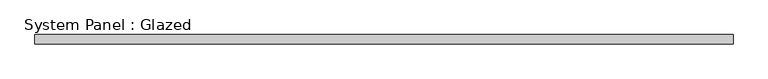
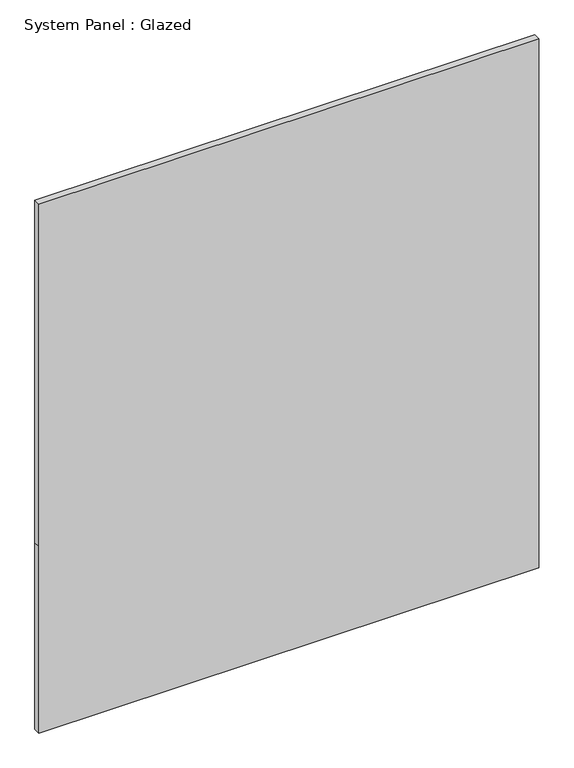
"""IFC4 building model written with IfcOpenShell, lengths in millimetres: plate geometry, System Panel : Glazed."""

import ifcopenshell
import ifcopenshell.guid

model = None  # the IFC model being written
_history = None  # IfcOwnerHistory: only IFC2X3 demands one
_inside = {}  # id of a spatial element -> (the spatial element, [elements in it])
_under = {}  # id of a project, library or spatial element -> (it, [spatial elements below it])
_declared = {}  # id of a project -> (the project, [libraries it declares])
_typed = {}  # id of a type object -> (the type object, [elements of that type])
_made_of = {}  # id of a material, layer set ... -> (it, [elements and type objects made of it])


def new_model(schema):
    """Start an empty IFC model of exactly this schema.

    Asked for "IFC4X3", IfcOpenShell would pick the latest addendum, in which some entities
    have other attributes; the version numbers below select the first issue.
    IFC2X3 requires an IfcOwnerHistory on every rooted entity: one is made here for all.
    """
    global model, _history
    if schema == "IFC4X3":
        model = ifcopenshell.file(schema_version=(4, 3, 0, 0))
    else:
        model = ifcopenshell.file(schema=schema)
    _inside.clear()
    _under.clear()
    _declared.clear()
    _typed.clear()
    _made_of.clear()
    _history = None
    if model.schema == "IFC2X3":
        org = make("IfcOrganization", Name="unknown")
        user = make(
            "IfcPersonAndOrganization",
            ThePerson=make("IfcPerson", FamilyName="unknown"),
            TheOrganization=org,
        )
        app = make(
            "IfcApplication",
            ApplicationDeveloper=org,
            Version="unknown",
            ApplicationFullName="unknown",
            ApplicationIdentifier="unknown",
        )
        _history = make(
            "IfcOwnerHistory",
            OwningUser=user,
            OwningApplication=app,
            ChangeAction="ADDED",
            CreationDate=0,
        )
    return model


def make(cls, **values):
    """One entity of the class cls with the attributes given. An attribute that is None is left unset."""
    return model.create_entity(
        cls, **{name: value for name, value in values.items() if value is not None}
    )


def rooted(cls, **values):
    """An entity with a GlobalId (a new one), such as an element, a storey or a relation."""
    return make(cls, GlobalId=ifcopenshell.guid.new(), OwnerHistory=_history, **values)


def si_unit(unit_type, name, prefix=None):
    """IfcSIUnit, for example si_unit("LENGTHUNIT", "METRE", prefix="MILLI")."""
    return make("IfcSIUnit", UnitType=unit_type, Prefix=prefix, Name=name)


def assignment(units):
    """IfcUnitAssignment: the units of a project."""
    return None if units is None else make("IfcUnitAssignment", Units=units)


def point(xyz):
    """IfcCartesianPoint."""
    return None if xyz is None else make("IfcCartesianPoint", Coordinates=xyz)


def direction(xyz):
    """IfcDirection."""
    return None if xyz is None else make("IfcDirection", DirectionRatios=xyz)


def frame(location, z_axis=None, x_axis=None):
    """IfcAxis2Placement3D, a coordinate frame: its origin and axes. An axis left out is left unset."""
    return make(
        "IfcAxis2Placement3D",
        Location=point(location),
        Axis=direction(z_axis),
        RefDirection=direction(x_axis),
    )


def origin():
    """The frame at (0, 0, 0) with its axes left unset."""
    return frame((0.0, 0.0, 0.0))


def place(relative_to, where):
    """IfcLocalPlacement: puts the frame where relative to a parent placement (None: the world)."""
    return make(
        "IfcLocalPlacement", PlacementRelTo=relative_to, RelativePlacement=where
    )


def context(
    kind, dimensions, precision=None, world=None, true_north=None, identifier=None
):
    """IfcGeometricRepresentationContext, for example the 3D "Model" context."""
    return make(
        "IfcGeometricRepresentationContext",
        ContextIdentifier=identifier,
        ContextType=kind,
        CoordinateSpaceDimension=dimensions,
        Precision=precision,
        WorldCoordinateSystem=world,
        TrueNorth=true_north,
    )


def project(units=None, contexts=None):
    """IfcProject with its units and contexts."""
    return rooted(
        "IfcProject",
        Name="project",
        RepresentationContexts=contexts,
        UnitsInContext=assignment(units),
    )


def spatial(cls, under=None, at=None, **own):
    """A site, building, storey or space (cls), placed at a placement, below another one or the project."""
    s = rooted(cls, ObjectPlacement=at, **own)
    if under is not None:
        _under.setdefault(under.id(), (under, []))[1].append(s)
    return s


def polyline(points):
    """IfcPolyline through the points."""
    return make("IfcPolyline", Points=[point(p) for p in points])


def outline(outer, holes=None, kind="AREA"):
    """IfcArbitraryClosedProfileDef: a profile drawn as a closed curve; with holes, ...WithVoids."""
    if holes is None:
        return make("IfcArbitraryClosedProfileDef", ProfileType=kind, OuterCurve=outer)
    return make(
        "IfcArbitraryProfileDefWithVoids",
        ProfileType=kind,
        OuterCurve=outer,
        InnerCurves=holes,
    )


def extrude(swept, where, along, depth):
    """IfcExtrudedAreaSolid: the profile swept, set in the frame where, extruded along a direction by depth."""
    return make(
        "IfcExtrudedAreaSolid",
        SweptArea=swept,
        Position=where,
        ExtrudedDirection=direction(along),
        Depth=depth,
    )


def shape(context_of_items, identifier, shape_type, items):
    """IfcShapeRepresentation: the items that make up one representation, for example the "Body"."""
    return make(
        "IfcShapeRepresentation",
        ContextOfItems=context_of_items,
        RepresentationIdentifier=identifier,
        RepresentationType=shape_type,
        Items=items,
    )


def source(mapping_origin, context_of_items, identifier, shape_type, items):
    """IfcRepresentationMap: a shape defined once, which mapped items show again and again."""
    return make(
        "IfcRepresentationMap",
        MappingOrigin=mapping_origin,
        MappedRepresentation=shape(context_of_items, identifier, shape_type, items),
    )


def transform(
    local_origin,
    x_axis=None,
    y_axis=None,
    z_axis=None,
    scale=None,
    scale2=None,
    scale3=None,
    uniform=True,
):
    """IfcCartesianTransformationOperator3D, or its non-uniform kind. x_axis, y_axis, z_axis: its Axis1, 2, 3."""
    if uniform:
        return make(
            "IfcCartesianTransformationOperator3D",
            Axis1=direction(x_axis),
            Axis2=direction(y_axis),
            LocalOrigin=point(local_origin),
            Scale=scale,
            Axis3=direction(z_axis),
        )
    return make(
        "IfcCartesianTransformationOperator3DnonUniform",
        Axis1=direction(x_axis),
        Axis2=direction(y_axis),
        LocalOrigin=point(local_origin),
        Scale=scale,
        Axis3=direction(z_axis),
        Scale2=scale2,
        Scale3=scale3,
    )


def mapped(mapping_source, mapping_target):
    """IfcMappedItem: shows the shape of a source again, moved by a transform."""
    return make(
        "IfcMappedItem", MappingSource=mapping_source, MappingTarget=mapping_target
    )


def made_of(thing, what):
    """Note that an element or type object is made of a material, layer set ...; save() writes the relation."""
    if what is not None:
        _made_of.setdefault(what.id(), (what, []))[1].append(thing)
    return thing


def element(
    cls,
    number,
    at=None,
    inside=None,
    cuts=None,
    type_object=None,
    material=None,
    context=None,
    identifier="Body",
    shape_type=None,
    held_by="IfcProductDefinitionShape",
    body=None,
    shapes=None,
    **own,
):
    """One element of the class cls, such as IfcWall. Its Tag is "e" and its number.

    at: its placement. inside: the storey or other place that contains it. cuts: it is an
    opening in that element (IfcRelVoidsElement). A single representation is given by context,
    identifier, shape_type and body (its items); several are given by shapes. held_by: the class
    of the entity that holds the representations. save() writes the other relations.
    """
    e = rooted(cls, Tag="e%d" % number, ObjectPlacement=at, **own)
    if body is not None:
        shapes = [shape(context, identifier, shape_type, body)]
    if shapes is not None:
        e.Representation = make(held_by, Representations=shapes)
    if inside is not None:
        _inside.setdefault(inside.id(), (inside, []))[1].append(e)
    if cuts is not None:
        rooted(
            "IfcRelVoidsElement", RelatingBuildingElement=cuts, RelatedOpeningElement=e
        )
    if type_object is not None:
        _typed.setdefault(type_object.id(), (type_object, []))[1].append(e)
    return made_of(e, material)


def aggregate(whole, parts):
    """IfcRelAggregates: a whole, such as a stair, and the parts it consists of."""
    return rooted("IfcRelAggregates", RelatingObject=whole, RelatedObjects=parts)


def save(model, path):
    """Write the relations noted so far, then the file.

    IfcRelAggregates (storeys below a building ...), IfcRelContainedInSpatialStructure (elements
    in a storey), IfcRelDefinesByType, IfcRelAssociatesMaterial and IfcRelDeclares: one each for
    every whole, place, type object, material and project.
    """
    for whole, parts in _under.values():
        aggregate(whole, parts)
    for where, things in _inside.values():
        rooted(
            "IfcRelContainedInSpatialStructure",
            RelatedElements=things,
            RelatingStructure=where,
        )
    for kind, things in _typed.values():
        rooted("IfcRelDefinesByType", RelatedObjects=things, RelatingType=kind)
    for what, things in _made_of.values():
        rooted("IfcRelAssociatesMaterial", RelatedObjects=things, RelatingMaterial=what)
    for by, libraries in _declared.values():
        rooted("IfcRelDeclares", RelatingContext=by, RelatedDefinitions=libraries)
    model.write(path)


def system_panel_glazed_635c0c9e(model_context):
    return source(origin(), model_context, "Body", "SweptSolid", [
        extrude(outline(polyline([(0.0, -949.9999998), (0.0, 949.9999998), (750.0, 949.9999998), (2125.0, 949.9999998), (2125.0, -949.9999998), (750.0, -949.9999998), (0.0, -949.9999998)])), frame((0.0, 24.5, 0.0), z_axis=(0.0, 1.0, 0.0), x_axis=(0.0, 0.0, 1.0)), (0.0, 0.0, 1.0), 25.0),
    ])


if __name__ == "__main__":
    model = new_model("IFC4")
    model_context = context("Model", 3, world=origin())
    ifc_project = project(units=[si_unit("LENGTHUNIT", "METRE", prefix="MILLI")], contexts=[model_context])
    site = spatial("IfcSite", under=ifc_project)
    building = spatial("IfcBuilding", under=site)
    placement = place(None, origin())
    system_panel_glazed_shape = system_panel_glazed_635c0c9e(model_context)
    element("IfcPlate", 1, ObjectType="System Panel : Glazed", at=placement, inside=building, context=model_context, shape_type="MappedRepresentation", body=[
        mapped(system_panel_glazed_shape, transform((0.0, 0.0, 0.0), x_axis=(1.0, 0.0, 0.0), y_axis=(0.0, 1.0, 0.0), z_axis=(0.0, 0.0, 1.0))),
    ])
    save(model, "model.ifc")

# Revit data of these elements
# Element 1 (IfcPlate, "System Panel : Glazed")
#   Materials on its faces: "Glass"
# Materials
#   "Glass": class "Glass", colour RGB 0 128 192, transparency 0.9
